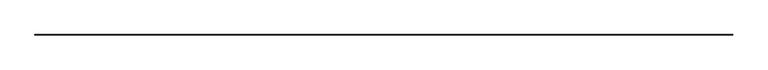
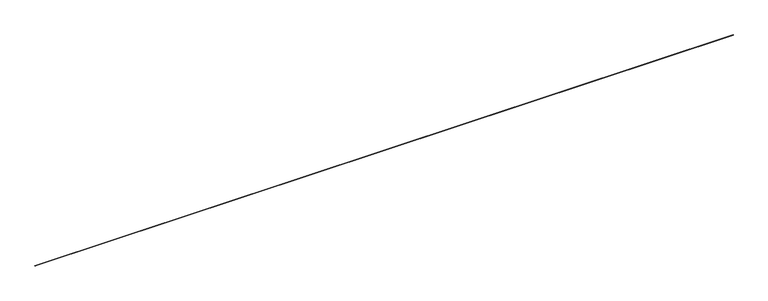
"""IFC4 building model written with IfcOpenShell, lengths in millimetres: proxy geometry, Inner panel:Inner panel:1:Inner panel:1 : Inner panel:Inner panel:300324:2:Inner panel:1:Inner panel:1 : Inner panel:Inner panel:300324:2 : Inner panel:Inner panel:1:Inner panel:1 : Inner panel:Inner panel:300324:300043:1 : Inner panel:Inner panel:1:Inner panel:1 : Inner panel:Inner panel:300324:2:Inner panel:1:Inner panel:1 : Inner panel:Inner panel:300324:2 : Inner panel:Inner panel:1:Inner panel:1 : Inner panel:Inner panel:300324:300043:308120."""

from ifc_helpers import new_model, si_unit, frame, origin, place, context, project, spatial, polyline, outline, extrude, source, transform, mapped, element, save


def generic_models_28c6dbaa(model_context):
    return source(origin(), model_context, "Body", "SweptSolid", [
        extrude(outline(polyline([(-569670.9723574, 8919.2746389), (-569653.0118451, 8937.2351512), (-569635.0513329, 8919.2746389), (-569653.0118451, 8901.3141267), (-569670.9723574, 8919.2746389)]), holes=[polyline([(-569667.6047613, 8919.2746389), (-569653.0118451, 8904.6817227), (-569638.4189289, 8919.2746389), (-569653.0118451, 8933.8675551), (-569667.6047613, 8919.2746389)])]), frame((579104.5117239, 0.0, 0.0), z_axis=(1.0, 0.0, 0.0), x_axis=(0.0, 1.0, 0.0)), (0.0, 0.0, 1.0), 88442.8),
    ])


if __name__ == "__main__":
    model = new_model("IFC4")
    model_context = context("Model", 3, world=origin())
    ifc_project = project(units=[si_unit("LENGTHUNIT", "METRE", prefix="MILLI")], contexts=[model_context])
    site = spatial("IfcSite", under=ifc_project)
    building = spatial("IfcBuilding", under=site)
    placement = place(None, origin())
    generic_models_shape = generic_models_28c6dbaa(model_context)
    element("IfcBuildingElementProxy", 1, Name="Inner panel:Inner panel:1:Inner panel:1 : Inner panel:Inner panel:300324:2:Inner panel:1:Inner panel:1 : Inner panel:Inner panel:300324:2 : Inner panel:Inner panel:1:Inner panel:1 : Inner panel:Inner panel:300324:300043:1 : Inner panel:Inner panel:1:Inner panel:1 : Inner panel:Inner panel:300324:2:Inner panel:1:Inner panel:1 : Inner panel:Inner panel:300324:2 : Inner panel:Inner panel:1:Inner panel:1 : Inner panel:Inner panel:300324:300043:308120", ObjectType="Inner panel:Inner panel:1:Inner panel:1 : Inner panel:Inner panel:300324:2:Inner panel:1:Inner panel:1 : Inner panel:Inner panel:300324:2 : Inner panel:Inner panel:1:Inner panel:1 : Inner panel:Inner panel:300324:300043:1 : Inner panel:Inner panel:1:Inner panel:1 : Inner panel:Inner panel:300324:2:Inner panel:1:Inner panel:1 : Inner panel:Inner panel:300324:2 : Inner panel:Inner panel:1:Inner panel:1 : Inner panel:Inner panel:300324:300043:308120", at=placement, inside=building, context=model_context, shape_type="MappedRepresentation", body=[
        mapped(generic_models_shape, transform((0.0, 0.0, 0.0), x_axis=(1.0, 0.0, 0.0), y_axis=(0.0, 1.0, 0.0), z_axis=(0.0, 0.0, 1.0))),
    ])
    save(model, "model.ifc")

# Revit data of these elements
# Type "Inner panel:Inner panel:1:Inner panel:1 : Inner panel:Inner panel:300324:2:Inner panel:1:Inner panel:1 : Inner panel:Inner panel:300324:2 : Inner panel:Inner panel:1:Inner panel:1 : Inner panel:Inner panel:300324:300043:1 : Inner panel:Inner panel:1:Inner panel:1 : Inner panel:Inner panel:300324:2:Inner panel:1:Inner panel:1 : Inner panel:Inner panel:300324:2 : Inner panel:Inner panel:1:Inner panel:1 : Inner panel:Inner panel:300324:300043:308120"
#   NameOverride = "Inner panel:Inner panel:1:Inner panel:1 : Inner panel:Inner panel:300324:2:Inner panel:1:Inner panel:1 : Inner panel:Inner panel:300324:2 : Inner panel:Inner panel:1:Inner panel:1 : Inner panel:Inner panel:300324:300043:308120"
#   ObjectTypeOverride = "Inner panel:1:Inner panel:1 : Inner panel:Inner panel:300324:2 : Inner panel:Inner panel:1:Inner panel:1 : Inner panel:Inner panel:300324:300043"
#   Reference = "Inner panel"
#   Tag = "308120"
# Element 1 (IfcBuildingElementProxy, "Inner panel:Inner panel:1:Inner panel:1 : Inner panel:Inner panel:300324:2:Inner panel:1:Inner panel:1 : Inner panel:Inner panel:300324:2 : Inner panel:Inner panel:1:Inner panel:1 : Inner panel:Inner panel:300324:300043:1 : Inner panel:Inner panel:1:Inner panel:1 : Inner panel:Inner panel:300324:2:Inner panel:1:Inner panel:1 : Inner panel:Inner panel:300324:2 : Inner panel:Inner panel:1:Inner panel:1 : Inner panel:Inner panel:300324:300043:308120")
#   Materials on its faces: "SNOW GUARD SYSTEM"
# Materials
#   "SNOW GUARD SYSTEM": class "Generic", colour RGB 223 223 223, transparency 0, Cost = 0
